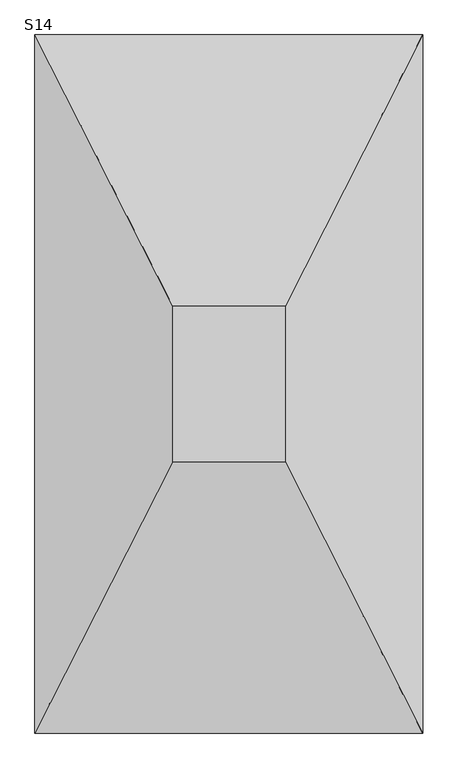
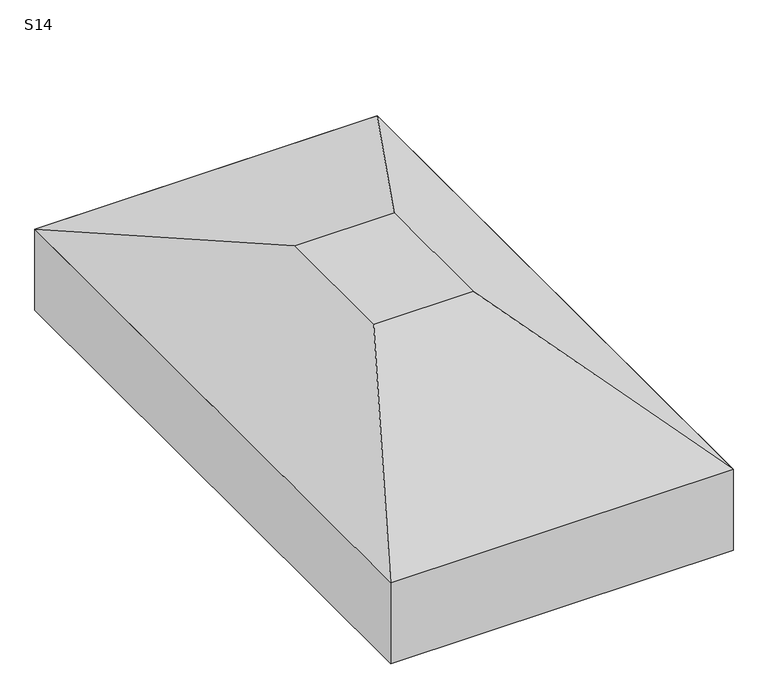
"""IFC4 building model written with IfcOpenShell, lengths in millimetres: fastener geometry, TQS - Sapata : S14."""

import ifcopenshell
import ifcopenshell.guid

model = None  # the IFC model being written
_history = None  # IfcOwnerHistory: only IFC2X3 demands one
_inside = {}  # id of a spatial element -> (the spatial element, [elements in it])
_under = {}  # id of a project, library or spatial element -> (it, [spatial elements below it])
_declared = {}  # id of a project -> (the project, [libraries it declares])
_typed = {}  # id of a type object -> (the type object, [elements of that type])
_made_of = {}  # id of a material, layer set ... -> (it, [elements and type objects made of it])


def new_model(schema):
    """Start an empty IFC model of exactly this schema.

    Asked for "IFC4X3", IfcOpenShell would pick the latest addendum, in which some entities
    have other attributes; the version numbers below select the first issue.
    IFC2X3 requires an IfcOwnerHistory on every rooted entity: one is made here for all.
    """
    global model, _history
    if schema == "IFC4X3":
        model = ifcopenshell.file(schema_version=(4, 3, 0, 0))
    else:
        model = ifcopenshell.file(schema=schema)
    _inside.clear()
    _under.clear()
    _declared.clear()
    _typed.clear()
    _made_of.clear()
    _history = None
    if model.schema == "IFC2X3":
        org = make("IfcOrganization", Name="unknown")
        user = make(
            "IfcPersonAndOrganization",
            ThePerson=make("IfcPerson", FamilyName="unknown"),
            TheOrganization=org,
        )
        app = make(
            "IfcApplication",
            ApplicationDeveloper=org,
            Version="unknown",
            ApplicationFullName="unknown",
            ApplicationIdentifier="unknown",
        )
        _history = make(
            "IfcOwnerHistory",
            OwningUser=user,
            OwningApplication=app,
            ChangeAction="ADDED",
            CreationDate=0,
        )
    return model


def make(cls, **values):
    """One entity of the class cls with the attributes given. An attribute that is None is left unset."""
    return model.create_entity(
        cls, **{name: value for name, value in values.items() if value is not None}
    )


def rooted(cls, **values):
    """An entity with a GlobalId (a new one), such as an element, a storey or a relation."""
    return make(cls, GlobalId=ifcopenshell.guid.new(), OwnerHistory=_history, **values)


def si_unit(unit_type, name, prefix=None):
    """IfcSIUnit, for example si_unit("LENGTHUNIT", "METRE", prefix="MILLI")."""
    return make("IfcSIUnit", UnitType=unit_type, Prefix=prefix, Name=name)


def assignment(units):
    """IfcUnitAssignment: the units of a project."""
    return None if units is None else make("IfcUnitAssignment", Units=units)


def point(xyz):
    """IfcCartesianPoint."""
    return None if xyz is None else make("IfcCartesianPoint", Coordinates=xyz)


def direction(xyz):
    """IfcDirection."""
    return None if xyz is None else make("IfcDirection", DirectionRatios=xyz)


def frame(location, z_axis=None, x_axis=None):
    """IfcAxis2Placement3D, a coordinate frame: its origin and axes. An axis left out is left unset."""
    return make(
        "IfcAxis2Placement3D",
        Location=point(location),
        Axis=direction(z_axis),
        RefDirection=direction(x_axis),
    )


def origin():
    """The frame at (0, 0, 0) with its axes left unset."""
    return frame((0.0, 0.0, 0.0))


def place(relative_to, where):
    """IfcLocalPlacement: puts the frame where relative to a parent placement (None: the world)."""
    return make(
        "IfcLocalPlacement", PlacementRelTo=relative_to, RelativePlacement=where
    )


def context(
    kind, dimensions, precision=None, world=None, true_north=None, identifier=None
):
    """IfcGeometricRepresentationContext, for example the 3D "Model" context."""
    return make(
        "IfcGeometricRepresentationContext",
        ContextIdentifier=identifier,
        ContextType=kind,
        CoordinateSpaceDimension=dimensions,
        Precision=precision,
        WorldCoordinateSystem=world,
        TrueNorth=true_north,
    )


def project(units=None, contexts=None):
    """IfcProject with its units and contexts."""
    return rooted(
        "IfcProject",
        Name="project",
        RepresentationContexts=contexts,
        UnitsInContext=assignment(units),
    )


def spatial(cls, under=None, at=None, **own):
    """A site, building, storey or space (cls), placed at a placement, below another one or the project."""
    s = rooted(cls, ObjectPlacement=at, **own)
    if under is not None:
        _under.setdefault(under.id(), (under, []))[1].append(s)
    return s


def polyline(points):
    """IfcPolyline through the points."""
    return make("IfcPolyline", Points=[point(p) for p in points])


def outline(outer, holes=None, kind="AREA"):
    """IfcArbitraryClosedProfileDef: a profile drawn as a closed curve; with holes, ...WithVoids."""
    if holes is None:
        return make("IfcArbitraryClosedProfileDef", ProfileType=kind, OuterCurve=outer)
    return make(
        "IfcArbitraryProfileDefWithVoids",
        ProfileType=kind,
        OuterCurve=outer,
        InnerCurves=holes,
    )


def extrude(swept, where, along, depth):
    """IfcExtrudedAreaSolid: the profile swept, set in the frame where, extruded along a direction by depth."""
    return make(
        "IfcExtrudedAreaSolid",
        SweptArea=swept,
        Position=where,
        ExtrudedDirection=direction(along),
        Depth=depth,
    )


def faces_of(points, faces, orient=None, outer=None):
    """IfcFace entities. A face is a list of loops; a loop is a list of indices into points, from 0.

    orient and outer hold one flag for each loop. By default every Orientation is true, the
    first loop of a face is its IfcFaceOuterBound and the others are IfcFaceBound.
    """
    made = []
    for i, loops in enumerate(faces):
        bounds = []
        for j, loop in enumerate(loops):
            is_outer = j == 0 if outer is None else outer[i][j]
            bounds.append(
                make(
                    "IfcFaceOuterBound" if is_outer else "IfcFaceBound",
                    Bound=make("IfcPolyLoop", Polygon=[points[k] for k in loop]),
                    Orientation=True if orient is None else orient[i][j],
                )
            )
        made.append(make("IfcFace", Bounds=bounds))
    return made


def faceted_brep(points, faces, orient=None, outer=None, voids=None):
    """IfcFacetedBrep: a solid bounded by flat faces; with voids (closed shells), ...WithVoids."""
    shared = [point(p) for p in points]
    hull = make("IfcClosedShell", CfsFaces=faces_of(shared, faces, orient, outer))
    if voids is None:
        return make("IfcFacetedBrep", Outer=hull)
    return make(
        "IfcFacetedBrepWithVoids",
        Outer=hull,
        Voids=[
            make(cls, CfsFaces=faces_of(shared, fs, o, b)) for cls, fs, o, b in voids
        ],
    )


def shape(context_of_items, identifier, shape_type, items):
    """IfcShapeRepresentation: the items that make up one representation, for example the "Body"."""
    return make(
        "IfcShapeRepresentation",
        ContextOfItems=context_of_items,
        RepresentationIdentifier=identifier,
        RepresentationType=shape_type,
        Items=items,
    )


def source(mapping_origin, context_of_items, identifier, shape_type, items):
    """IfcRepresentationMap: a shape defined once, which mapped items show again and again."""
    return make(
        "IfcRepresentationMap",
        MappingOrigin=mapping_origin,
        MappedRepresentation=shape(context_of_items, identifier, shape_type, items),
    )


def transform(
    local_origin,
    x_axis=None,
    y_axis=None,
    z_axis=None,
    scale=None,
    scale2=None,
    scale3=None,
    uniform=True,
):
    """IfcCartesianTransformationOperator3D, or its non-uniform kind. x_axis, y_axis, z_axis: its Axis1, 2, 3."""
    if uniform:
        return make(
            "IfcCartesianTransformationOperator3D",
            Axis1=direction(x_axis),
            Axis2=direction(y_axis),
            LocalOrigin=point(local_origin),
            Scale=scale,
            Axis3=direction(z_axis),
        )
    return make(
        "IfcCartesianTransformationOperator3DnonUniform",
        Axis1=direction(x_axis),
        Axis2=direction(y_axis),
        LocalOrigin=point(local_origin),
        Scale=scale,
        Axis3=direction(z_axis),
        Scale2=scale2,
        Scale3=scale3,
    )


def mapped(mapping_source, mapping_target):
    """IfcMappedItem: shows the shape of a source again, moved by a transform."""
    return make(
        "IfcMappedItem", MappingSource=mapping_source, MappingTarget=mapping_target
    )


def made_of(thing, what):
    """Note that an element or type object is made of a material, layer set ...; save() writes the relation."""
    if what is not None:
        _made_of.setdefault(what.id(), (what, []))[1].append(thing)
    return thing


def element(
    cls,
    number,
    at=None,
    inside=None,
    cuts=None,
    type_object=None,
    material=None,
    context=None,
    identifier="Body",
    shape_type=None,
    held_by="IfcProductDefinitionShape",
    body=None,
    shapes=None,
    **own,
):
    """One element of the class cls, such as IfcWall. Its Tag is "e" and its number.

    at: its placement. inside: the storey or other place that contains it. cuts: it is an
    opening in that element (IfcRelVoidsElement). A single representation is given by context,
    identifier, shape_type and body (its items); several are given by shapes. held_by: the class
    of the entity that holds the representations. save() writes the other relations.
    """
    e = rooted(cls, Tag="e%d" % number, ObjectPlacement=at, **own)
    if body is not None:
        shapes = [shape(context, identifier, shape_type, body)]
    if shapes is not None:
        e.Representation = make(held_by, Representations=shapes)
    if inside is not None:
        _inside.setdefault(inside.id(), (inside, []))[1].append(e)
    if cuts is not None:
        rooted(
            "IfcRelVoidsElement", RelatingBuildingElement=cuts, RelatedOpeningElement=e
        )
    if type_object is not None:
        _typed.setdefault(type_object.id(), (type_object, []))[1].append(e)
    return made_of(e, material)


def aggregate(whole, parts):
    """IfcRelAggregates: a whole, such as a stair, and the parts it consists of."""
    return rooted("IfcRelAggregates", RelatingObject=whole, RelatedObjects=parts)


def save(model, path):
    """Write the relations noted so far, then the file.

    IfcRelAggregates (storeys below a building ...), IfcRelContainedInSpatialStructure (elements
    in a storey), IfcRelDefinesByType, IfcRelAssociatesMaterial and IfcRelDeclares: one each for
    every whole, place, type object, material and project.
    """
    for whole, parts in _under.values():
        aggregate(whole, parts)
    for where, things in _inside.values():
        rooted(
            "IfcRelContainedInSpatialStructure",
            RelatedElements=things,
            RelatingStructure=where,
        )
    for kind, things in _typed.values():
        rooted("IfcRelDefinesByType", RelatedObjects=things, RelatingType=kind)
    for what, things in _made_of.values():
        rooted("IfcRelAssociatesMaterial", RelatedObjects=things, RelatingMaterial=what)
    for by, libraries in _declared.values():
        rooted("IfcRelDeclares", RelatingContext=by, RelatedDefinitions=libraries)
    model.write(path)


def s14_8166d2be(model_context):
    return source(origin(), model_context, "Body", "SolidModel", [
        faceted_brep([(-55.0, 0.0, 0.0), (-345.0, 0.0, 0.0), (-345.0, -400.0, 0.0), (-55.0, -400.0, 0.0), (300.0, 700.0, -250.0), (300.0, -1100.0, -250.0), (-700.0, -1100.0, -250.0), (-700.0, 700.0, -250.0)], [[[0, 1, 2, 3]], [[4, 5, 6, 7]], [[4, 7, 1, 0]], [[7, 6, 2, 1]], [[6, 5, 3, 2]], [[5, 4, 0, 3]]]),
        extrude(outline(polyline([(300.0, 700.0), (300.0, -1100.0), (-700.0, -1100.0), (-700.0, 700.0), (300.0, 700.0)])), frame((0.0, 0.0, -500.0), z_axis=(0.0, 0.0, 1.0), x_axis=(1.0, 0.0, 0.0)), (0.0, 0.0, 1.0), 250.0),
    ])


if __name__ == "__main__":
    model = new_model("IFC4")
    model_context = context("Model", 3, world=origin())
    ifc_project = project(units=[si_unit("LENGTHUNIT", "METRE", prefix="MILLI")], contexts=[model_context])
    site = spatial("IfcSite", under=ifc_project)
    building = spatial("IfcBuilding", under=site)
    placement = place(None, origin())
    s14_shape = s14_8166d2be(model_context)
    element("IfcFastener", 1, ObjectType="TQS - Sapata : S14", at=placement, inside=building, context=model_context, shape_type="MappedRepresentation", body=[
        mapped(s14_shape, transform((0.0, 0.0, 0.0), x_axis=(1.0, 0.0, 0.0), y_axis=(0.0, 1.0, 0.0), z_axis=(0.0, 0.0, 1.0))),
    ])
    save(model, "model.ifc")

# Revit data of these elements
# Type "TQS - Sapata : S14"
#   TY = 0.40 m
#   TX = 0.29 m
#   HS = 0.50 m
#   H0 = 0.25 m
#   EXCYABS = 0.90 m
#   EXCY = 0.00 m
#   EXCXABS = 0.50 m
#   EXCX = 0.00 m
#   DIMY = 1.80 m
#   DIMX = 1.00 m
#   Material estrutural = Concreto - Concreto concretado no local
#   Width = 0
#   Length = 0
# Element 1 (IfcFastener, "TQS - Sapata : S14")
#   Materials on its faces: "Concreto - Concreto concretado no local"
# Materials
#   "Concreto - Concreto concretado no local": class "Concreto", colour RGB 192 192 192, transparency 0
